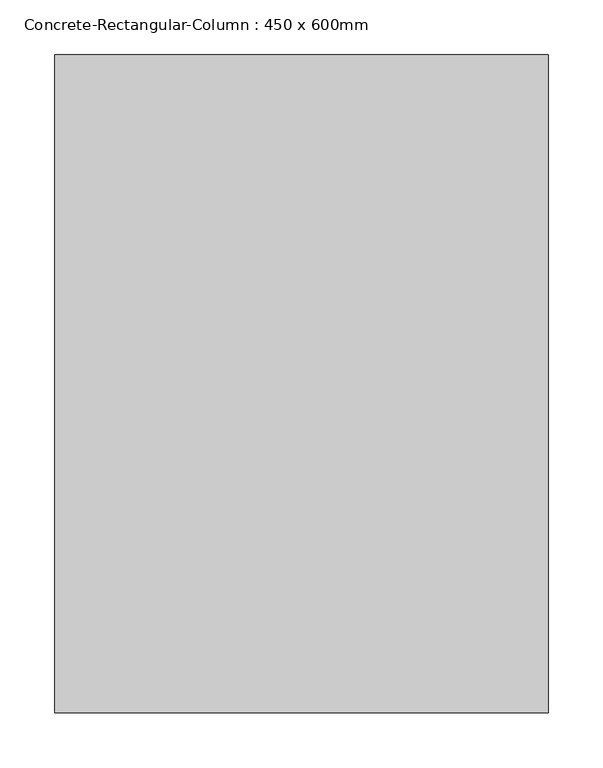
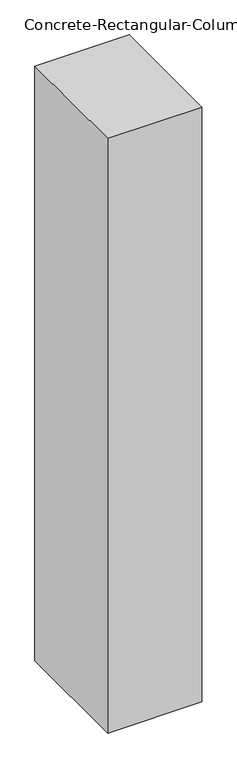
"""IFC4 building model written with IfcOpenShell, lengths in millimetres: column geometry, Concrete-Rectangular-Column : 450 x 600mm."""

from ifc_helpers import new_model, si_unit, origin, origin_with_axes, place, context, project, spatial, polyline, outline, extrude, source, transform, mapped, element, save


def concrete_rectangular_column_450_x_600mm_2b408faa(model_context):
    return source(origin(), model_context, "Body", "SweptSolid", [
        extrude(outline(polyline([(225.0, 300.0), (225.0, -300.0), (-225.0, -300.0), (-225.0, 300.0), (225.0, 300.0)])), origin_with_axes(), (0.0, 0.0, 1.0), 3000.0),
    ])


if __name__ == "__main__":
    model = new_model("IFC4")
    model_context = context("Model", 3, world=origin())
    ifc_project = project(units=[si_unit("LENGTHUNIT", "METRE", prefix="MILLI")], contexts=[model_context])
    site = spatial("IfcSite", under=ifc_project)
    building = spatial("IfcBuilding", under=site)
    placement = place(None, origin())
    concrete_rectangular_column_450_x_600mm_shape = concrete_rectangular_column_450_x_600mm_2b408faa(model_context)
    element("IfcColumn", 1, ObjectType="Concrete-Rectangular-Column : 450 x 600mm", at=placement, inside=building, context=model_context, shape_type="MappedRepresentation", body=[
        mapped(concrete_rectangular_column_450_x_600mm_shape, transform((0.0, 0.0, 0.0), x_axis=(1.0, 0.0, 0.0), y_axis=(0.0, 1.0, 0.0), z_axis=(0.0, 0.0, 1.0))),
    ])
    save(model, "model.ifc")

# Revit data of these elements
# Type "Concrete-Rectangular-Column : 450 x 600mm"
#   b = 450 mm
#   h = 600 mm
#   Structural Material [instance default] = none
# Element 1 (IfcColumn, "Concrete-Rectangular-Column : 450 x 600mm")
#   Structural Material = Concrete - Cast-in-Place Concrete - C30/37
#   Materials on its faces: "Concrete - Cast-in-Place Concrete - C30/37"
# Materials
#   "Concrete - Cast-in-Place Concrete - C30/37": class "Unassigned", colour RGB 192 192 192, transparency 0
